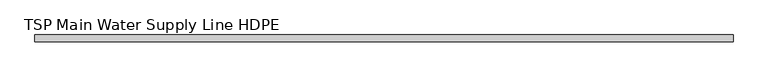
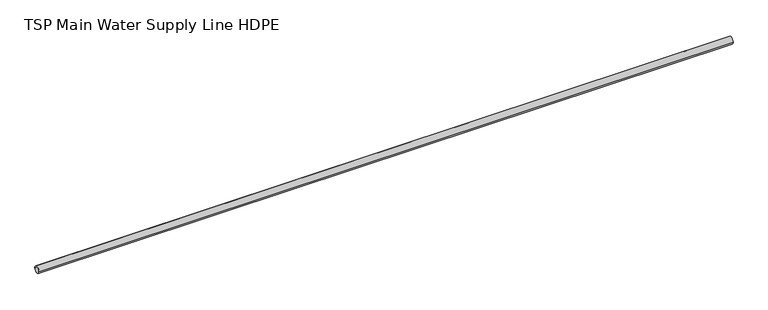
"""IFC4 building model written with IfcOpenShell, lengths in millimetres: flow terminal geometry, TSP Main Water Supply Line HDPE : HDPE Fresh Water Supply."""

from ifc_helpers import new_model, si_unit, point, frame, origin, origin_2d, place, context, project, spatial, circle_curve, trimmed, segment, composite_curve, outline, extrude, source, transform, mapped, element, save


def tsp_main_water_supply_line_hdpe_14c14526(model_context):
    return source(origin(), model_context, "Body", "SweptSolid", [
        extrude(outline(composite_curve([segment(trimmed(circle_curve(origin_2d(), 16.0), [point((-16.0, 0.0))], [point((16.0, 0.0))], False, "CARTESIAN"), True, "CONTINUOUS"), segment(trimmed(circle_curve(origin_2d(), 16.0), [point((16.0, 0.0))], [point((-16.0, 0.0))], False, "CARTESIAN"), True, "CONTINUOUS")], self_intersect=False), holes=[composite_curve([segment(trimmed(circle_curve(origin_2d(), 15.0), [point((-15.0, 0.0))], [point((15.0, 0.0))], True, "CARTESIAN"), True, "CONTINUOUS"), segment(trimmed(circle_curve(origin_2d(), 15.0), [point((15.0, 0.0))], [point((-15.0, 0.0))], True, "CARTESIAN"), True, "CONTINUOUS")], self_intersect=False)]), frame((0.0, 0.0, 0.0), z_axis=(1.0, 0.0, 0.0), x_axis=(0.0, 1.0, 0.0)), (0.0, 0.0, 1.0), 3166.2282021),
    ])


if __name__ == "__main__":
    model = new_model("IFC4")
    model_context = context("Model", 3, world=origin())
    ifc_project = project(units=[si_unit("LENGTHUNIT", "METRE", prefix="MILLI")], contexts=[model_context])
    site = spatial("IfcSite", under=ifc_project)
    building = spatial("IfcBuilding", under=site)
    placement = place(None, origin())
    tsp_main_water_supply_line_hdpe_shape = tsp_main_water_supply_line_hdpe_14c14526(model_context)
    element("IfcFlowTerminal", 1, ObjectType="TSP Main Water Supply Line HDPE : HDPE Fresh Water Supply", at=placement, inside=building, context=model_context, shape_type="MappedRepresentation", body=[
        mapped(tsp_main_water_supply_line_hdpe_shape, transform((0.0, 0.0, 0.0), x_axis=(1.0, 0.0, 0.0), y_axis=(0.0, 1.0, 0.0), z_axis=(0.0, 0.0, 1.0))),
    ])
    save(model, "model.ifc")

# Revit data of these elements
# Type "TSP Main Water Supply Line HDPE : HDPE Fresh Water Supply"
#   Model = "TSP_110SFWSP"
#   Pipe length [instance default] = 1200 mm
#   Pipe dia = 30 mm
#   built-in parameter 1001306 [instance default] = 3.93701 (stored number, unit not read)
#   Default Elevation = 0
# Element 1 (IfcFlowTerminal, "TSP Main Water Supply Line HDPE : HDPE Fresh Water Supply")
#   Pipe length = 3166.228 mm
#   built-in parameter 1001306 = 10.3879 (stored number, unit not read)
#   Materials on its faces: "Aluminum, Anodized Blue"
# Materials
#   "Aluminum, Anodized Blue": class "Metal", colour RGB 120 120 120, transparency 0, Description = "Anodized aluminum, blue", Cost = 0
